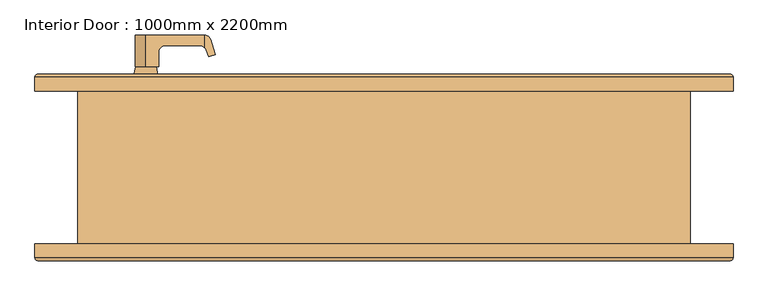
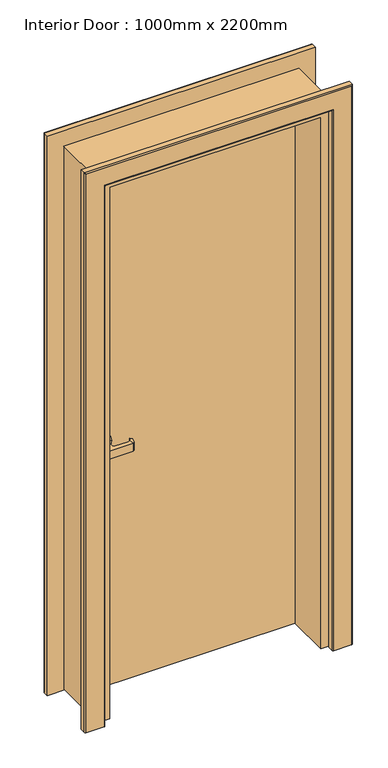
"""IFC4 building model written with IfcOpenShell, lengths in millimetres: door geometry, Interior Door : 1000mm x 2200mm."""

from ifc_helpers import new_model, si_unit, frame, origin, place, context, project, spatial, polyline, circle_curve, ellipse_curve, outline, extrude, faceted_brep, source, transform, mapped, element, save
from ifc_brep_helpers import plane_surface, cylinder_surface, revolved_surface, advanced_brep


def interior_door_1000mm_x_2200mm_5ae40eff(model_context):
    return source(origin(), model_context, "Body", "SolidModel", [
        advanced_brep(
        [(-323.0, 55.325, 910.0), (-377.0, 55.325, 910.0), (-368.0, 55.325, 910.0), (-332.0, 55.325, 910.0), (-349.5, 55.325, 922.0), (-350.5, 55.325, 922.0), (-350.5, 55.325, 898.0), (-349.5, 55.325, 898.0), (-323.0, 58.5, 910.0), (-377.0, 58.5, 910.0), (-332.0, 43.9713587, 910.0), (-368.0, 43.9713587, 910.0), (-349.5, 43.9713587, 898.0), (-350.5, 43.9713587, 898.0), (-350.5, 43.9713587, 922.0), (-349.5, 43.9713587, 922.0)],
        [
            (0, 1, circle_curve(frame((-350.0, 55.325, 910.0), z_axis=(0.0, -1.0, 0.0), x_axis=(-1.0, 0.0, 0.0)), 27.0)),
            (1, 0, circle_curve(frame((-350.0, 55.325, 910.0), z_axis=(0.0, -1.0, 0.0), x_axis=(-1.0, 0.0, 0.0)), 27.0)),
            (2, 3, circle_curve(frame((-350.0, 55.325, 910.0), z_axis=(0.0, 1.0, 0.0), x_axis=(-1.0, 0.0, 0.0)), 18.0)),
            (3, 2, circle_curve(frame((-350.0, 55.325, 910.0), z_axis=(0.0, 1.0, 0.0), x_axis=(-1.0, 0.0, 0.0)), 18.0)),
            (4, 5),
            (5, 6),
            (6, 7),
            (7, 4),
            (8, 9, circle_curve(frame((-350.0, 58.5, 910.0), z_axis=(0.0, 1.0, 0.0), x_axis=(-1.0, 0.0, 0.0)), 27.0)),
            (9, 8, circle_curve(frame((-350.0, 58.5, 910.0), z_axis=(0.0, 1.0, 0.0), x_axis=(-1.0, 0.0, 0.0)), 27.0)),
            (1, 9),
            (8, 0),
            (10, 11, circle_curve(frame((-350.0, 43.9713587, 910.0), z_axis=(0.0, -1.0, 0.0), x_axis=(-1.0, 0.0, 0.0)), 18.0)),
            (11, 10, circle_curve(frame((-350.0, 43.9713587, 910.0), z_axis=(0.0, -1.0, 0.0), x_axis=(-1.0, 0.0, 0.0)), 18.0)),
            (12, 13),
            (13, 14),
            (14, 15),
            (15, 12),
            (11, 2),
            (3, 10),
            (15, 4),
            (7, 12),
            (14, 5),
            (13, 6),
        ],
        [
            plane_surface(frame((-377.0, 55.325, 910.0), z_axis=(0.0, -1.0, 0.0), x_axis=(0.0, 0.0, 1.0))),
            plane_surface(frame((-377.0, 58.5, 910.0), z_axis=(0.0, 1.0, 0.0), x_axis=(0.0, 0.0, -1.0))),
            cylinder_surface(frame((-350.0, 58.5, 910.0), z_axis=(0.0, -1.0, 0.0), x_axis=(-1.0, 0.0, 0.0)), 27.0),
            plane_surface(frame((-368.0, 43.9713587, 910.0), z_axis=(0.0, -1.0, 0.0), x_axis=(0.0, 0.0, 1.0))),
            cylinder_surface(frame((-350.0, 58.5, 910.0), z_axis=(0.0, -1.0, 0.0), x_axis=(-1.0, 0.0, 0.0)), 18.0),
            plane_surface(frame((-349.5, 43.9713587, 898.0), z_axis=(-1.0, 0.0, 0.0), x_axis=(0.0, 1.0, 0.0))),
            plane_surface(frame((-349.5, 43.9713587, 922.0), z_axis=(0.0, 0.0, -1.0), x_axis=(0.0, 1.0, 0.0))),
            plane_surface(frame((-350.5, 43.9713587, 922.0), z_axis=(1.0, 0.0, 0.0), x_axis=(0.0, 1.0, 0.0))),
            plane_surface(frame((-350.5, 43.9713587, 898.0), z_axis=(0.0, 0.0, 1.0), x_axis=(0.0, 1.0, 0.0))),
        ],
        [
            (0, [[1, 2], [3, 4]]),
            (0, [[5, 6, 7, 8]]),
            (1, [[9, 10]]),
            (2, [[11, -9, 12, -2]]),
            (2, [[-12, -10, -11, -1]]),
            (3, [[13, 14], [15, 16, 17, 18]]),
            (4, [[19, -4, 20, -14]]),
            (4, [[-20, -3, -19, -13]]),
            (5, [[21, -8, 22, -18]]),
            (6, [[23, -5, -21, -17]]),
            (7, [[24, -6, -23, -16]]),
            (8, [[-22, -7, -24, -15]]),
        ],
    ),
        advanced_brep(
        [(-323.0, 115.675, 910.0), (-377.0, 115.675, 910.0), (-368.0, 115.675, 910.0), (-332.0, 115.675, 910.0), (-349.5, 115.675, 922.0), (-349.5, 115.675, 898.0), (-350.5, 115.675, 898.0), (-350.5, 115.675, 922.0), (-323.0, 112.5, 910.0), (-377.0, 112.5, 910.0), (-332.0, 127.0286413, 910.0), (-368.0, 127.0286413, 910.0), (-349.5, 127.0286413, 898.0), (-349.5, 127.0286413, 922.0), (-350.5, 127.0286413, 922.0), (-350.5, 127.0286413, 898.0)],
        [
            (0, 1, circle_curve(frame((-350.0, 115.675, 910.0), z_axis=(0.0, 1.0, 0.0), x_axis=(-1.0, 0.0, 0.0)), 27.0)),
            (1, 0, circle_curve(frame((-350.0, 115.675, 910.0), z_axis=(0.0, 1.0, 0.0), x_axis=(-1.0, 0.0, 0.0)), 27.0)),
            (2, 3, circle_curve(frame((-350.0, 115.675, 910.0), z_axis=(0.0, -1.0, 0.0), x_axis=(-1.0, 0.0, 0.0)), 18.0)),
            (3, 2, circle_curve(frame((-350.0, 115.675, 910.0), z_axis=(0.0, -1.0, 0.0), x_axis=(-1.0, 0.0, 0.0)), 18.0)),
            (4, 5),
            (5, 6),
            (6, 7),
            (7, 4),
            (8, 9, circle_curve(frame((-350.0, 112.5, 910.0), z_axis=(0.0, -1.0, 0.0), x_axis=(-1.0, 0.0, 0.0)), 27.0)),
            (9, 8, circle_curve(frame((-350.0, 112.5, 910.0), z_axis=(0.0, -1.0, 0.0), x_axis=(-1.0, 0.0, 0.0)), 27.0)),
            (0, 8),
            (9, 1),
            (10, 11, circle_curve(frame((-350.0, 127.0286413, 910.0), z_axis=(0.0, 1.0, 0.0), x_axis=(-1.0, 0.0, 0.0)), 18.0)),
            (11, 10, circle_curve(frame((-350.0, 127.0286413, 910.0), z_axis=(0.0, 1.0, 0.0), x_axis=(-1.0, 0.0, 0.0)), 18.0)),
            (12, 13),
            (13, 14),
            (14, 15),
            (15, 12),
            (10, 3),
            (2, 11),
            (12, 5),
            (4, 13),
            (7, 14),
            (6, 15),
        ],
        [
            plane_surface(frame((-377.0, 115.675, 910.0), z_axis=(0.0, 1.0, 0.0), x_axis=(0.0, 0.0, 1.0))),
            plane_surface(frame((-377.0, 112.5, 910.0), z_axis=(0.0, -1.0, 0.0), x_axis=(0.0, 0.0, -1.0))),
            cylinder_surface(frame((-350.0, 112.5, 910.0), z_axis=(0.0, 1.0, 0.0), x_axis=(-1.0, 0.0, 0.0)), 27.0),
            plane_surface(frame((-368.0, 127.0286413, 910.0), z_axis=(0.0, 1.0, 0.0), x_axis=(0.0, 0.0, 1.0))),
            cylinder_surface(frame((-350.0, 112.5, 910.0), z_axis=(0.0, 1.0, 0.0), x_axis=(-1.0, 0.0, 0.0)), 18.0),
            plane_surface(frame((-349.5, 127.0286413, 898.0), z_axis=(-1.0, 0.0, 0.0), x_axis=(0.0, -1.0, 0.0))),
            plane_surface(frame((-349.5, 127.0286413, 922.0), z_axis=(0.0, 0.0, -1.0), x_axis=(0.0, -1.0, 0.0))),
            plane_surface(frame((-350.5, 127.0286413, 922.0), z_axis=(1.0, 0.0, 0.0), x_axis=(0.0, -1.0, 0.0))),
            plane_surface(frame((-350.5, 127.0286413, 898.0), z_axis=(0.0, 0.0, 1.0), x_axis=(0.0, -1.0, 0.0))),
        ],
        [
            (0, [[1, 2], [3, 4]]),
            (0, [[5, 6, 7, 8]]),
            (1, [[9, 10]]),
            (2, [[-1, 11, -10, 12]]),
            (2, [[-2, -12, -9, -11]]),
            (3, [[13, 14], [15, 16, 17, 18]]),
            (4, [[-13, 19, -3, 20]]),
            (4, [[-14, -20, -4, -19]]),
            (5, [[-15, 21, -5, 22]]),
            (6, [[-16, -22, -8, 23]]),
            (7, [[-17, -23, -7, 24]]),
            (8, [[-18, -24, -6, -21]]),
        ],
    ),
        advanced_brep(
        [(-305.55, 125.2, 1000.0), (-305.55, 112.5, 1000.0), (-394.45, 112.5, 1000.0), (-394.45, 125.2, 1000.0), (-330.95, 128.375, 1000.0), (-369.05, 128.375, 1000.0), (-350.0, 112.5, 1000.0), (-334.9229513, 148.8140625, 1000.0), (-365.0770487, 148.8140625, 1000.0), (-350.0, 148.8140625, 1000.0)],
        [
            (0, 1),
            (1, 2, circle_curve(frame((-350.0, 112.5, 1000.0), z_axis=(0.0, 1.0, 0.0), x_axis=(-1.0, 0.0, 0.0)), 44.45)),
            (2, 3),
            (3, 0, circle_curve(frame((-350.0, 125.2, 1000.0), z_axis=(0.0, -1.0, 0.0), x_axis=(-1.0, 0.0, 0.0)), 44.45)),
            (2, 1, circle_curve(frame((-350.0, 112.5, 1000.0), z_axis=(0.0, 1.0, 0.0), x_axis=(-1.0, 0.0, 0.0)), 44.45)),
            (0, 3, circle_curve(frame((-350.0, 125.2, 1000.0), z_axis=(0.0, -1.0, 0.0), x_axis=(-1.0, 0.0, 0.0)), 44.45)),
            (4, 0),
            (3, 5),
            (5, 4, circle_curve(frame((-350.0, 128.375, 1000.0), z_axis=(0.0, -1.0, 0.0), x_axis=(-1.0, 0.0, 0.0)), 19.05)),
            (4, 5, circle_curve(frame((-350.0, 128.375, 1000.0), z_axis=(0.0, -1.0, 0.0), x_axis=(-1.0, 0.0, 0.0)), 19.05)),
            (1, 6),
            (6, 2),
            (7, 4),
            (5, 8),
            (8, 7, circle_curve(frame((-350.0, 148.8140625, 1000.0), z_axis=(0.0, -1.0, 0.0), x_axis=(-1.0, 0.0, 0.0)), 15.0770487)),
            (7, 8, circle_curve(frame((-350.0, 148.8140625, 1000.0), z_axis=(0.0, -1.0, 0.0), x_axis=(-1.0, 0.0, 0.0)), 15.0770487)),
            (9, 7),
            (8, 9),
        ],
        [
            cylinder_surface(frame((-350.0, -39.9, 1000.0), z_axis=(0.0, 1.0, 0.0), x_axis=(-1.0, 0.0, 0.0)), 44.45),
            revolved_surface(polyline([(-394.45, 125.2, 1000.0), (-369.05, 128.375, 1000.0)]), (-350.0, -39.9, 1000.0), (0.0, 1.0, 0.0)),
            plane_surface(frame((-350.0, 112.5, 1000.0), z_axis=(0.0, -1.0, 0.0), x_axis=(-1.0, 0.0, 0.0))),
            revolved_surface(polyline([(-369.05, 128.375, 1000.0), (-365.0770487, 148.8140625, 1000.0)]), (-350.0, -39.9, 1000.0), (0.0, 1.0, 0.0)),
            plane_surface(frame((-350.0, 148.8140625, 1000.0), z_axis=(0.0, 1.0, 0.0), x_axis=(-1.0, 0.0, 0.0))),
        ],
        [
            (0, [[1, 2, 3, 4]]),
            (0, [[-3, 5, -1, 6]]),
            (1, [[7, -4, 8, 9]]),
            (1, [[-8, -6, -7, 10]]),
            (2, [[11, 12, -2]]),
            (2, [[-12, -11, -5]]),
            (3, [[13, -9, 14, 15]]),
            (3, [[-14, -10, -13, 16]]),
            (4, [[17, -15, 18]]),
            (4, [[-18, -16, -17]]),
        ],
    ),
        advanced_brep(
        [(-330.95, 169.7736937, 1015.875), (-321.425, 179.2986937, 1015.875), (-270.4853465, 179.2986937, 1015.875), (-264.0071516, 176.7564308, 1015.875), (-264.0071516, 195.05, 1015.875), (-350.0, 195.05, 1015.875), (-350.0, 148.8140625, 1015.875), (-330.95, 148.8140625, 1015.875), (-330.95, 169.7736937, 984.125), (-330.95, 148.8140625, 984.125), (-350.0, 148.8140625, 984.125), (-350.0, 195.05, 984.125), (-264.0071516, 195.05, 984.125), (-264.0071516, 176.7564308, 984.125), (-270.4853465, 179.2986937, 984.125), (-321.425, 179.2986937, 984.125), (-261.5347742, 173.0314356, 984.7111937), (-261.5347742, 173.0314356, 1015.2888063), (-257.8148231, 162.8109537, 985.5931836), (-257.8148231, 162.8109537, 1014.4068164), (-247.6815328, 166.1034593, 987.9957581), (-247.6815328, 166.1034593, 1012.0042419), (-254.9483383, 188.4683869, 986.272819), (-254.9483383, 188.4683869, 1013.727181)],
        [
            (0, 1, circle_curve(frame((-321.425, 169.7736937, 1015.875), z_axis=(0.0, 0.0, -1.0), x_axis=(1.0, 0.0, 0.0)), 9.525)),
            (1, 2),
            (2, 3, circle_curve(frame((-270.4853465, 169.7736937, 1015.875), z_axis=(0.0, 0.0, -1.0), x_axis=(1.0, 0.0, 0.0)), 9.525)),
            (3, 4),
            (4, 5),
            (5, 6),
            (6, 7),
            (7, 0),
            (8, 9),
            (9, 10),
            (10, 11),
            (11, 12),
            (12, 13),
            (13, 14, circle_curve(frame((-270.4853465, 169.7736937, 984.125), z_axis=(0.0, 0.0, 1.0), x_axis=(1.0, 0.0, 0.0)), 9.525)),
            (14, 15),
            (15, 8, circle_curve(frame((-321.425, 169.7736937, 984.125), z_axis=(0.0, 0.0, 1.0), x_axis=(1.0, 0.0, 0.0)), 9.525)),
            (7, 9),
            (8, 0),
            (1, 15),
            (14, 2),
            (11, 5, circle_curve(frame((-350.0, 195.05, 1000.0), z_axis=(0.0, 1.0, 0.0), x_axis=(0.0, 0.0, 1.0)), 15.875)),
            (4, 12),
            (6, 10, circle_curve(frame((-350.0, 148.8140625, 1000.0), z_axis=(0.0, -1.0, 0.0), x_axis=(0.0, 0.0, 1.0)), 15.875)),
            (13, 16, ellipse_curve(frame((-270.4853465, 169.7736937, 982.5890383), z_axis=(0.23070138294863055, 0.0, -0.9730245998460623), x_axis=(0.9730245998460625, 0.0, 0.23070138294862935)), 9.7890639, 9.525)),
            (16, 17),
            (17, 3, ellipse_curve(frame((-270.4853465, 169.7736937, 1017.4109617), z_axis=(0.23070138294863687, 0.0, 0.9730245998460607), x_axis=(-0.9730245998460608, 0.0, 0.23070138294863632)), 9.7890639, 9.525)),
            (16, 18),
            (18, 19),
            (19, 17),
            (18, 20),
            (20, 21),
            (21, 19),
            (20, 22),
            (22, 23),
            (23, 21),
            (4, 23, ellipse_curve(frame((-264.0071516, 185.525, 1015.875), z_axis=(-0.23070138294863687, 0.0, -0.9730245998460607), x_axis=(0.9730245998460608, 0.0, -0.23070138294863632)), 9.7890639, 9.525)),
            (22, 12, ellipse_curve(frame((-264.0071516, 185.525, 984.125), z_axis=(-0.23070138294863055, 0.0, 0.9730245998460623), x_axis=(-0.9730245998460625, 0.0, -0.23070138294862935)), 9.7890639, 9.525)),
        ],
        [
            plane_surface(frame((-311.9, 169.7736937, 1015.875), z_axis=(0.0, 0.0, 1.0), x_axis=(0.0, 1.0, 0.0))),
            plane_surface(frame((-311.9, 169.7736937, 984.125), z_axis=(0.0, 0.0, -1.0), x_axis=(0.0, -1.0, 0.0))),
            plane_surface(frame((-330.95, 148.8140625, 984.125), z_axis=(1.0, 0.0, 0.0), x_axis=(0.0, 0.0, 1.0))),
            plane_surface(frame((-321.425, 179.2986937, 984.125), z_axis=(0.0, -1.0, 0.0), x_axis=(0.0, 0.0, 1.0))),
            plane_surface(frame((-264.0071516, 195.05, 984.125), z_axis=(0.0, 1.0, 0.0), x_axis=(0.0, 0.0, 1.0))),
            plane_surface(frame((-369.05, 148.8140625, 984.125), z_axis=(0.0, -1.0, 0.0), x_axis=(0.0, 0.0, 1.0))),
            revolved_surface(polyline([(-311.90000000000003, 169.7736937, 1015.875), (-311.90000000000003, 169.7736937, 984.125)]), (-321.425, 169.7736937, 1015.875), (0.0, 0.0, 1.0)),
            revolved_surface(polyline([(-260.9603465, 169.7736937, 1019.6693122795026), (-260.9603465, 169.7736937, 980.3306877204975)]), (-270.4853465, 169.7736937, 1015.875), (0.0, 0.0, 1.0)),
            plane_surface(frame((-261.5347742, 173.0314356, 984.125), z_axis=(-0.93969262078591, -0.3420201433256644, 0.0), x_axis=(0.0, 0.0, 1.0))),
            plane_surface(frame((-257.8148231, 162.8109537, 984.125), z_axis=(0.30901699437494523, -0.9510565162951543, 0.0), x_axis=(0.0, 0.0, 1.0))),
            plane_surface(frame((-247.6815328, 166.1034593, 984.125), z_axis=(0.9510565162951542, 0.3090169943749457, 0.0), x_axis=(0.0, 0.0, 1.0))),
            cylinder_surface(frame((-264.0071516, 185.525, 1015.875), z_axis=(0.0, 0.0, -1.0), x_axis=(1.0, 0.0, 0.0)), 9.525),
            cylinder_surface(frame((-350.0, 417.3, 1000.0), z_axis=(0.0, 1.0, 0.0), x_axis=(0.0, 0.0, 1.0)), 15.875),
            plane_surface(frame((-264.0071516, -192.3, 984.125), z_axis=(0.23070138294863055, 0.0, -0.9730245998460623), x_axis=(0.0, 1.0, 0.0))),
            plane_surface(frame((-236.70001, -192.3, 1009.4005539), z_axis=(0.23070138294863687, 0.0, 0.9730245998460607), x_axis=(0.0, 1.0, 0.0))),
        ],
        [
            (0, [[1, 2, 3, 4, 5, 6, 7, 8]]),
            (1, [[9, 10, 11, 12, 13, 14, 15, 16]]),
            (2, [[17, -9, 18, -8]]),
            (3, [[19, -15, 20, -2]]),
            (4, [[-12, 21, -5, 22]]),
            (5, [[-7, 23, -10, -17]]),
            (6, [[-18, -16, -19, -1]]),
            (7, [[-14, 24, 25, 26, -3, -20]]),
            (8, [[27, 28, 29, -25]]),
            (9, [[30, 31, 32, -28]]),
            (10, [[33, 34, 35, -31]]),
            (11, [[36, -34, 37, -22]]),
            (12, [[-21, -11, -23, -6]]),
            (13, [[-37, -33, -30, -27, -24, -13]]),
            (14, [[-26, -29, -32, -35, -36, -4]]),
        ],
    ),
        advanced_brep(
        [(-305.55, 45.8, 1000.0), (-394.45, 45.8, 1000.0), (-394.45, 58.5, 1000.0), (-305.55, 58.5, 1000.0), (-330.95, 42.625, 1000.0), (-369.05, 42.625, 1000.0), (-350.0, 58.5, 1000.0), (-334.9229513, 22.1859375, 1000.0), (-365.0770487, 22.1859375, 1000.0), (-350.0, 22.1859375, 1000.0)],
        [
            (0, 1, circle_curve(frame((-350.0, 45.8, 1000.0), z_axis=(0.0, 1.0, 0.0), x_axis=(-1.0, 0.0, 0.0)), 44.45)),
            (1, 2),
            (2, 3, circle_curve(frame((-350.0, 58.5, 1000.0), z_axis=(0.0, -1.0, 0.0), x_axis=(-1.0, 0.0, 0.0)), 44.45)),
            (3, 0),
            (1, 0, circle_curve(frame((-350.0, 45.8, 1000.0), z_axis=(0.0, 1.0, 0.0), x_axis=(-1.0, 0.0, 0.0)), 44.45)),
            (3, 2, circle_curve(frame((-350.0, 58.5, 1000.0), z_axis=(0.0, -1.0, 0.0), x_axis=(-1.0, 0.0, 0.0)), 44.45)),
            (4, 5, circle_curve(frame((-350.0, 42.625, 1000.0), z_axis=(0.0, 1.0, 0.0), x_axis=(-1.0, 0.0, 0.0)), 19.05)),
            (5, 1),
            (0, 4),
            (5, 4, circle_curve(frame((-350.0, 42.625, 1000.0), z_axis=(0.0, 1.0, 0.0), x_axis=(-1.0, 0.0, 0.0)), 19.05)),
            (2, 6),
            (6, 3),
            (7, 8, circle_curve(frame((-350.0, 22.1859375, 1000.0), z_axis=(0.0, 1.0, 0.0), x_axis=(-1.0, 0.0, 0.0)), 15.0770487)),
            (8, 5),
            (4, 7),
            (8, 7, circle_curve(frame((-350.0, 22.1859375, 1000.0), z_axis=(0.0, 1.0, 0.0), x_axis=(-1.0, 0.0, 0.0)), 15.0770487)),
            (9, 8),
            (7, 9),
        ],
        [
            cylinder_surface(frame((-350.0, 210.9, 1000.0), z_axis=(0.0, -1.0, 0.0), x_axis=(-1.0, 0.0, 0.0)), 44.45),
            revolved_surface(polyline([(-394.45, 45.8, 1000.0), (-369.05, 42.625, 1000.0)]), (-350.0, 210.9, 1000.0), (0.0, -1.0, 0.0)),
            plane_surface(frame((-350.0, 58.5, 1000.0), z_axis=(0.0, 1.0, 0.0), x_axis=(-1.0, 0.0, 0.0))),
            revolved_surface(polyline([(-369.05, 42.625, 1000.0), (-365.0770487, 22.1859375, 1000.0)]), (-350.0, 210.9, 1000.0), (0.0, -1.0, 0.0)),
            plane_surface(frame((-350.0, 22.1859375, 1000.0), z_axis=(0.0, -1.0, 0.0), x_axis=(-1.0, 0.0, 0.0))),
        ],
        [
            (0, [[1, 2, 3, 4]]),
            (0, [[5, -4, 6, -2]]),
            (1, [[7, 8, -1, 9]]),
            (1, [[10, -9, -5, -8]]),
            (2, [[-3, 11, 12]]),
            (2, [[-6, -12, -11]]),
            (3, [[13, 14, -7, 15]]),
            (3, [[16, -15, -10, -14]]),
            (4, [[17, -13, 18]]),
            (4, [[-18, -16, -17]]),
        ],
    ),
        advanced_brep(
        [(-330.95, 1.2263063, 1015.875), (-330.95, 22.1859375, 1015.875), (-350.0, 22.1859375, 1015.875), (-350.0, -24.05, 1015.875), (-264.0071516, -24.05, 1015.875), (-264.0071516, -5.7564308, 1015.875), (-270.4853465, -8.2986937, 1015.875), (-321.425, -8.2986937, 1015.875), (-330.95, 1.2263063, 984.125), (-321.425, -8.2986937, 984.125), (-270.4853465, -8.2986937, 984.125), (-264.0071516, -5.7564308, 984.125), (-264.0071516, -24.05, 984.125), (-350.0, -24.05, 984.125), (-350.0, 22.1859375, 984.125), (-330.95, 22.1859375, 984.125), (-261.5347742, -2.0314356, 1015.2888063), (-261.5347742, -2.0314356, 984.7111937), (-257.8148231, 8.1890463, 1014.4068164), (-257.8148231, 8.1890463, 985.5931836), (-247.6815328, 4.8965407, 1012.0042419), (-247.6815328, 4.8965407, 987.9957581), (-254.9483383, -17.4683869, 1013.727181), (-254.9483383, -17.4683869, 986.272819)],
        [
            (0, 1),
            (1, 2),
            (2, 3),
            (3, 4),
            (4, 5),
            (5, 6, circle_curve(frame((-270.4853465, 1.2263063, 1015.875), z_axis=(0.0, 0.0, -1.0), x_axis=(1.0, 0.0, 0.0)), 9.525)),
            (6, 7),
            (7, 0, circle_curve(frame((-321.425, 1.2263063, 1015.875), z_axis=(0.0, 0.0, -1.0), x_axis=(1.0, 0.0, 0.0)), 9.525)),
            (8, 9, circle_curve(frame((-321.425, 1.2263063, 984.125), z_axis=(0.0, 0.0, 1.0), x_axis=(1.0, 0.0, 0.0)), 9.525)),
            (9, 10),
            (10, 11, circle_curve(frame((-270.4853465, 1.2263063, 984.125), z_axis=(0.0, 0.0, 1.0), x_axis=(1.0, 0.0, 0.0)), 9.525)),
            (11, 12),
            (12, 13),
            (13, 14),
            (14, 15),
            (15, 8),
            (0, 8),
            (15, 1),
            (6, 10),
            (9, 7),
            (12, 4),
            (3, 13, circle_curve(frame((-350.0, -24.05, 1000.0), z_axis=(0.0, -1.0, 0.0), x_axis=(0.0, 0.0, 1.0)), 15.875)),
            (14, 2, circle_curve(frame((-350.0, 22.1859375, 1000.0), z_axis=(0.0, 1.0, 0.0), x_axis=(0.0, 0.0, 1.0)), 15.875)),
            (5, 16, ellipse_curve(frame((-270.4853465, 1.2263063, 1017.4109617), z_axis=(0.23070138294863687, 0.0, 0.9730245998460607), x_axis=(-0.9730245998460608, 0.0, 0.23070138294863632)), 9.7890639, 9.525)),
            (16, 17),
            (17, 11, ellipse_curve(frame((-270.4853465, 1.2263063, 982.5890383), z_axis=(0.23070138294863055, 0.0, -0.9730245998460623), x_axis=(0.9730245998460625, 0.0, 0.23070138294862935)), 9.7890639, 9.525)),
            (16, 18),
            (18, 19),
            (19, 17),
            (18, 20),
            (20, 21),
            (21, 19),
            (20, 22),
            (22, 23),
            (23, 21),
            (12, 23, ellipse_curve(frame((-264.0071516, -14.525, 984.125), z_axis=(-0.23070138294863055, 0.0, 0.9730245998460623), x_axis=(-0.9730245998460625, 0.0, -0.23070138294862935)), 9.7890639, 9.525)),
            (22, 4, ellipse_curve(frame((-264.0071516, -14.525, 1015.875), z_axis=(-0.23070138294863687, 0.0, -0.9730245998460607), x_axis=(0.9730245998460608, 0.0, -0.23070138294863632)), 9.7890639, 9.525)),
        ],
        [
            plane_surface(frame((-311.9, 1.2263063, 1015.875), z_axis=(0.0, 0.0, 1.0), x_axis=(0.0, -1.0, 0.0))),
            plane_surface(frame((-311.9, 1.2263063, 984.125), z_axis=(0.0, 0.0, -1.0), x_axis=(0.0, 1.0, 0.0))),
            plane_surface(frame((-330.95, 22.1859375, 984.125), z_axis=(1.0, 0.0, 0.0), x_axis=(0.0, 0.0, 1.0))),
            plane_surface(frame((-321.425, -8.2986937, 984.125), z_axis=(0.0, 1.0, 0.0), x_axis=(0.0, 0.0, 1.0))),
            plane_surface(frame((-264.0071516, -24.05, 984.125), z_axis=(0.0, -1.0, 0.0), x_axis=(0.0, 0.0, 1.0))),
            plane_surface(frame((-369.05, 22.1859375, 984.125), z_axis=(0.0, 1.0, 0.0), x_axis=(0.0, 0.0, 1.0))),
            revolved_surface(polyline([(-311.90000000000003, 1.2263063, 1015.875), (-311.90000000000003, 1.2263063, 984.125)]), (-321.425, 1.2263063, 1015.875), (0.0, 0.0, 1.0)),
            revolved_surface(polyline([(-260.9603465, 1.2263063, 1019.6693122795026), (-260.9603465, 1.2263063, 980.3306877204975)]), (-270.4853465, 1.2263063, 1015.875), (0.0, 0.0, 1.0)),
            plane_surface(frame((-261.5347742, -2.0314356, 984.125), z_axis=(-0.93969262078591, 0.3420201433256644, 0.0), x_axis=(0.0, 0.0, 1.0))),
            plane_surface(frame((-257.8148231, 8.1890463, 984.125), z_axis=(0.30901699437494523, 0.9510565162951543, 0.0), x_axis=(0.0, 0.0, 1.0))),
            plane_surface(frame((-247.6815328, 4.8965407, 984.125), z_axis=(0.9510565162951542, -0.3090169943749457, 0.0), x_axis=(0.0, 0.0, 1.0))),
            cylinder_surface(frame((-264.0071516, -14.525, 1015.875), z_axis=(0.0, 0.0, -1.0), x_axis=(1.0, 0.0, 0.0)), 9.525),
            cylinder_surface(frame((-350.0, -246.3, 1000.0), z_axis=(0.0, -1.0, 0.0), x_axis=(0.0, 0.0, 1.0)), 15.875),
            plane_surface(frame((-264.0071516, 363.3, 984.125), z_axis=(0.23070138294863055, 0.0, -0.9730245998460623), x_axis=(0.0, -1.0, 0.0))),
            plane_surface(frame((-236.70001, 363.3, 1009.4005539), z_axis=(0.23070138294863687, 0.0, 0.9730245998460607), x_axis=(0.0, -1.0, 0.0))),
        ],
        [
            (0, [[1, 2, 3, 4, 5, 6, 7, 8]]),
            (1, [[9, 10, 11, 12, 13, 14, 15, 16]]),
            (2, [[-1, 17, -16, 18]]),
            (3, [[-7, 19, -10, 20]]),
            (4, [[21, -4, 22, -13]]),
            (5, [[-18, -15, 23, -2]]),
            (6, [[-8, -20, -9, -17]]),
            (7, [[-19, -6, 24, 25, 26, -11]]),
            (8, [[-25, 27, 28, 29]]),
            (9, [[-28, 30, 31, 32]]),
            (10, [[-31, 33, 34, 35]]),
            (11, [[-21, 36, -34, 37]]),
            (12, [[-3, -23, -14, -22]]),
            (13, [[-12, -26, -29, -32, -35, -36]]),
            (14, [[-5, -37, -33, -30, -27, -24]]),
        ],
    ),
        extrude(outline(polyline([(422.0000374, 58.5), (-422.0000374, 58.5), (-422.0000374, 112.5), (422.0000374, 112.5), (422.0000374, 58.5)])), frame((0.0, 0.0, 5.0), z_axis=(0.0, 0.0, 1.0), x_axis=(1.0, 0.0, 0.0)), (0.0, 0.0, 1.0), 2167.0000374),
        faceted_brep([(-405.0000128, 58.5, 5.0), (-405.0000128, -112.5, 5.0), (-450.0, -112.5, 5.0), (-450.0, 112.5, 5.0), (-422.0000374, 112.5, 5.0), (-422.0000374, 58.5, 5.0), (-405.0000128, 58.5, 2155.0000128), (-405.0000128, -112.5, 2155.0000128), (405.0000128, -112.5, 2155.0000128), (405.0000128, -112.5, 5.0), (450.0, -112.5, 5.0), (450.0, -112.5, 2200.0), (-450.0, -112.5, 2200.0), (-450.0, 112.5, 2200.0), (450.0, 112.5, 2200.0), (450.0, 112.5, 5.0), (422.0000374, 112.5, 5.0), (422.0000374, 112.5, 2172.0000374), (-422.0000374, 112.5, 2172.0000374), (-422.0000374, 58.5, 2172.0000374), (422.0000374, 58.5, 2172.0000374), (422.0000374, 58.5, 5.0), (405.0000128, 58.5, 5.0), (405.0000128, 58.5, 2155.0000128)], [[[0, 1, 2, 3, 4, 5]], [[0, 6, 7, 1]], [[2, 1, 7, 8, 9, 10, 11, 12]], [[3, 2, 12, 13]], [[4, 3, 13, 14, 15, 16, 17, 18]], [[5, 4, 18, 19]], [[0, 5, 19, 20, 21, 22, 23, 6]], [[8, 23, 22, 9]], [[9, 22, 21, 16, 15, 10]], [[14, 11, 10, 15]], [[20, 17, 16, 21]], [[13, 12, 11, 14]], [[19, 18, 17, 20]], [[7, 6, 23, 8]]]),
        advanced_brep(
        [(-439.9983436, 137.5, 0.0), (-435.0, 132.5016564, 0.0), (-435.0, 112.5, 0.0), (-512.9993919, 112.5, 0.0), (-512.9993919, 132.4992678, 0.0), (-507.9986597, 137.5, 0.0), (-439.9983436, 137.5, 2189.9983436), (-435.0, 132.5016564, 2185.0), (-435.0, 112.5, 2185.0), (435.0, 112.5, 2185.0), (435.0, 112.5, 0.0), (512.9993919, 112.5, 0.0), (512.9993919, 112.5, 2262.9993919), (-512.9993919, 112.5, 2262.9993919), (-512.9993919, 132.4992678, 2262.9993919), (-507.9986597, 137.5, 2257.9986597), (507.9986597, 137.5, 2257.9986597), (507.9986597, 137.5, 0.0), (439.9983436, 137.5, 0.0), (439.9983436, 137.5, 2189.9983436), (435.0, 132.5016564, 2185.0), (435.0, 132.5016564, 0.0), (512.9993919, 132.4992678, 0.0), (512.9993919, 132.4992678, 2262.9993919)],
        [
            (0, 1, circle_curve(frame((-439.9983436, 132.5016564, 0.0), z_axis=(0.0, 0.0, -1.0), x_axis=(-1.0, 0.0, 0.0)), 4.9983436)),
            (1, 2),
            (2, 3),
            (3, 4),
            (4, 5, circle_curve(frame((-507.9986597, 132.4992678, 0.0), z_axis=(0.0, 0.0, -1.0), x_axis=(-1.0, 0.0, 0.0)), 5.0007322)),
            (5, 0),
            (0, 6),
            (6, 7, ellipse_curve(frame((-439.9983436, 132.5016564, 2189.9983436), z_axis=(-0.7071067811865475, 0.0, -0.7071067811865475), x_axis=(0.7071067811865474, 0.0, -0.7071067811865476)), 7.0687253, 4.9983436)),
            (7, 1),
            (7, 8),
            (8, 2),
            (8, 9),
            (9, 10),
            (10, 11),
            (11, 12),
            (12, 13),
            (13, 3),
            (13, 14),
            (14, 4),
            (14, 15, ellipse_curve(frame((-507.9986597, 132.4992678, 2257.9986597), z_axis=(-0.7071067811865475, 0.0, -0.7071067811865475), x_axis=(0.7071067811865474, 0.0, -0.7071067811865476)), 7.0721032, 5.0007322)),
            (15, 5),
            (15, 16),
            (16, 17),
            (17, 18),
            (18, 19),
            (19, 6),
            (9, 20),
            (20, 21),
            (21, 10),
            (17, 22, circle_curve(frame((507.9986597, 132.4992678, 0.0), z_axis=(0.0, 0.0, -1.0), x_axis=(1.0, 0.0, 0.0)), 5.0007322)),
            (22, 11),
            (21, 18, circle_curve(frame((439.9983436, 132.5016564, 0.0), z_axis=(0.0, 0.0, -1.0), x_axis=(1.0, 0.0, 0.0)), 4.9983436)),
            (23, 12),
            (22, 23),
            (16, 23, ellipse_curve(frame((507.9986597, 132.4992678, 2257.9986597), z_axis=(0.7071067811865475, 0.0, -0.7071067811865475), x_axis=(0.7071067811865474, 0.0, 0.7071067811865476)), 7.0721032, 5.0007322)),
            (20, 19, ellipse_curve(frame((439.9983436, 132.5016564, 2189.9983436), z_axis=(0.7071067811865475, 0.0, -0.7071067811865475), x_axis=(0.7071067811865474, 0.0, 0.7071067811865476)), 7.0687253, 4.9983436)),
            (20, 7),
            (23, 14),
        ],
        [
            plane_surface(frame((-450.0, -125.0, 0.0), z_axis=(0.0, 0.0, -1.0), x_axis=(0.0, -1.0, 0.0))),
            cylinder_surface(frame((-439.9983436, 132.5016564, 0.0), z_axis=(0.0, 0.0, -1.0), x_axis=(-1.0, 0.0, 0.0)), 4.9983436),
            plane_surface(frame((-435.0, 132.5016564, 0.0), z_axis=(1.0, 0.0, 0.0), x_axis=(0.0, 0.0, 1.0))),
            plane_surface(frame((-435.0, 112.5, 0.0), z_axis=(0.0, -1.0, 0.0), x_axis=(0.0, 0.0, 1.0))),
            plane_surface(frame((-512.9993919, 112.5, 0.0), z_axis=(-1.0, 0.0, 0.0), x_axis=(0.0, 0.0, 1.0))),
            cylinder_surface(frame((-507.9986597, 132.4992678, 0.0), z_axis=(0.0, 0.0, -1.0), x_axis=(-1.0, 0.0, 0.0)), 5.0007322),
            plane_surface(frame((-507.9986597, 137.5, 0.0), z_axis=(0.0, 1.0, 0.0), x_axis=(0.0, 0.0, 1.0))),
            plane_surface(frame((435.0, 132.5016564, 2185.0), z_axis=(-1.0, 0.0, 0.0), x_axis=(0.0, 0.0, -1.0))),
            plane_surface(frame((450.0, -125.0, 0.0), z_axis=(0.0, 0.0, -1.0), x_axis=(0.0, -1.0, 0.0))),
            plane_surface(frame((512.9993919, 112.5, 2262.9993919), z_axis=(1.0, 0.0, 0.0), x_axis=(0.0, 0.0, -1.0))),
            cylinder_surface(frame((507.9986597, 132.4992678, 2200.0), z_axis=(0.0, 0.0, 1.0), x_axis=(1.0, 0.0, 0.0)), 5.0007322),
            cylinder_surface(frame((439.9983436, 132.5016564, 2200.0), z_axis=(0.0, 0.0, 1.0), x_axis=(1.0, 0.0, 0.0)), 4.9983436),
            cylinder_surface(frame((-450.0, 132.5016564, 2189.9983436), z_axis=(-1.0, 0.0, 0.0), x_axis=(0.0, 0.0, 1.0)), 4.9983436),
            plane_surface(frame((-435.0, 132.5016564, 2185.0), z_axis=(0.0, 0.0, -1.0), x_axis=(1.0, 0.0, 0.0))),
            plane_surface(frame((-512.9993919, 112.5, 2262.9993919), z_axis=(0.0, 0.0, 1.0), x_axis=(1.0, 0.0, 0.0))),
            cylinder_surface(frame((-450.0, 132.4992678, 2257.9986597), z_axis=(-1.0, 0.0, 0.0), x_axis=(0.0, 0.0, 1.0)), 5.0007322),
        ],
        [
            (0, [[1, 2, 3, 4, 5, 6]]),
            (1, [[-1, 7, 8, 9]]),
            (2, [[-2, -9, 10, 11]]),
            (3, [[-3, -11, 12, 13, 14, 15, 16, 17]]),
            (4, [[-4, -17, 18, 19]]),
            (5, [[-5, -19, 20, 21]]),
            (6, [[-6, -21, 22, 23, 24, 25, 26, -7]]),
            (7, [[27, 28, 29, -13]]),
            (8, [[-24, 30, 31, -14, -29, 32]]),
            (9, [[33, -15, -31, 34]]),
            (10, [[35, -34, -30, -23]]),
            (11, [[36, -25, -32, -28]]),
            (12, [[-8, -26, -36, 37]]),
            (13, [[-10, -37, -27, -12]]),
            (14, [[-18, -16, -33, 38]]),
            (15, [[-20, -38, -35, -22]]),
        ],
    ),
        advanced_brep(
        [(-439.9983436, -137.5, 0.0), (-507.9986597, -137.5, 0.0), (-512.9993919, -132.4992678, 0.0), (-512.9993919, -112.5, 0.0), (-435.0, -112.5, 0.0), (-435.0, -132.5016564, 0.0), (-439.9983436, -137.5, 2189.9983436), (439.9983436, -137.5, 2189.9983436), (439.9983436, -137.5, 0.0), (507.9986597, -137.5, 0.0), (507.9986597, -137.5, 2257.9986597), (-507.9986597, -137.5, 2257.9986597), (-512.9993919, -132.4992678, 2262.9993919), (-512.9993919, -112.5, 2262.9993919), (512.9993919, -112.5, 2262.9993919), (512.9993919, -112.5, 0.0), (435.0, -112.5, 0.0), (435.0, -112.5, 2185.0), (-435.0, -112.5, 2185.0), (-435.0, -132.5016564, 2185.0), (512.9993919, -132.4992678, 2262.9993919), (512.9993919, -132.4992678, 0.0), (435.0, -132.5016564, 0.0), (435.0, -132.5016564, 2185.0)],
        [
            (0, 1),
            (1, 2, circle_curve(frame((-507.9986597, -132.4992678, 0.0), z_axis=(0.0, 0.0, -1.0), x_axis=(1.0, 0.0, 0.0)), 5.0007322)),
            (2, 3),
            (3, 4),
            (4, 5),
            (5, 0, circle_curve(frame((-439.9983436, -132.5016564, 0.0), z_axis=(0.0, 0.0, -1.0), x_axis=(1.0, 0.0, 0.0)), 4.9983436)),
            (0, 6),
            (6, 7),
            (7, 8),
            (8, 9),
            (9, 10),
            (10, 11),
            (11, 1),
            (11, 12, ellipse_curve(frame((-507.9986597, -132.4992678, 2257.9986597), z_axis=(-0.7071067811865475, 0.0, -0.7071067811865475), x_axis=(0.7071067811865474, 0.0, -0.7071067811865476)), 7.0721032, 5.0007322)),
            (12, 2),
            (12, 13),
            (13, 3),
            (13, 14),
            (14, 15),
            (15, 16),
            (16, 17),
            (17, 18),
            (18, 4),
            (18, 19),
            (19, 5),
            (19, 6, ellipse_curve(frame((-439.9983436, -132.5016564, 2189.9983436), z_axis=(-0.7071067811865475, 0.0, -0.7071067811865475), x_axis=(0.7071067811865474, 0.0, -0.7071067811865476)), 7.0687253, 4.9983436)),
            (14, 20),
            (20, 21),
            (21, 15),
            (8, 22, circle_curve(frame((439.9983436, -132.5016564, 0.0), z_axis=(0.0, 0.0, -1.0), x_axis=(-1.0, 0.0, 0.0)), 4.9983436)),
            (22, 16),
            (21, 9, circle_curve(frame((507.9986597, -132.4992678, 0.0), z_axis=(0.0, 0.0, -1.0), x_axis=(-1.0, 0.0, 0.0)), 5.0007322)),
            (23, 17),
            (22, 23),
            (7, 23, ellipse_curve(frame((439.9983436, -132.5016564, 2189.9983436), z_axis=(0.7071067811865475, 0.0, -0.7071067811865475), x_axis=(0.7071067811865474, 0.0, 0.7071067811865476)), 7.0687253, 4.9983436)),
            (20, 10, ellipse_curve(frame((507.9986597, -132.4992678, 2257.9986597), z_axis=(0.7071067811865475, 0.0, -0.7071067811865475), x_axis=(0.7071067811865474, 0.0, 0.7071067811865476)), 7.0721032, 5.0007322)),
            (19, 23),
            (12, 20),
        ],
        [
            plane_surface(frame((-450.0, 125.0, 0.0), z_axis=(0.0, 0.0, -1.0), x_axis=(0.0, 1.0, 0.0))),
            plane_surface(frame((-439.9983436, -137.5, 0.0), z_axis=(0.0, -1.0, 0.0), x_axis=(0.0, 0.0, 1.0))),
            cylinder_surface(frame((-507.9986597, -132.4992678, 0.0), z_axis=(0.0, 0.0, -1.0), x_axis=(1.0, 0.0, 0.0)), 5.0007322),
            plane_surface(frame((-512.9993919, -132.4992678, 0.0), z_axis=(-1.0, 0.0, 0.0), x_axis=(0.0, 0.0, 1.0))),
            plane_surface(frame((-512.9993919, -112.5, 0.0), z_axis=(0.0, 1.0, 0.0), x_axis=(0.0, 0.0, 1.0))),
            plane_surface(frame((-435.0, -112.5, 0.0), z_axis=(1.0, 0.0, 0.0), x_axis=(0.0, 0.0, 1.0))),
            cylinder_surface(frame((-439.9983436, -132.5016564, 0.0), z_axis=(0.0, 0.0, -1.0), x_axis=(1.0, 0.0, 0.0)), 4.9983436),
            plane_surface(frame((512.9993919, -132.4992678, 2262.9993919), z_axis=(1.0, 0.0, 0.0), x_axis=(0.0, 0.0, -1.0))),
            plane_surface(frame((450.0, 125.0, 0.0), z_axis=(0.0, 0.0, -1.0), x_axis=(0.0, 1.0, 0.0))),
            plane_surface(frame((435.0, -112.5, 2185.0), z_axis=(-1.0, 0.0, 0.0), x_axis=(0.0, 0.0, -1.0))),
            cylinder_surface(frame((439.9983436, -132.5016564, 2200.0), z_axis=(0.0, 0.0, 1.0), x_axis=(-1.0, 0.0, 0.0)), 4.9983436),
            cylinder_surface(frame((507.9986597, -132.4992678, 2200.0), z_axis=(0.0, 0.0, 1.0), x_axis=(-1.0, 0.0, 0.0)), 5.0007322),
            cylinder_surface(frame((-450.0, -132.5016564, 2189.9983436), z_axis=(-1.0, 0.0, 0.0), x_axis=(0.0, 0.0, -1.0)), 4.9983436),
            plane_surface(frame((-435.0, -112.5, 2185.0), z_axis=(0.0, 0.0, -1.0), x_axis=(1.0, 0.0, 0.0))),
            plane_surface(frame((-512.9993919, -132.4992678, 2262.9993919), z_axis=(0.0, 0.0, 1.0), x_axis=(1.0, 0.0, 0.0))),
            cylinder_surface(frame((-450.0, -132.4992678, 2257.9986597), z_axis=(-1.0, 0.0, 0.0), x_axis=(0.0, 0.0, -1.0)), 5.0007322),
        ],
        [
            (0, [[1, 2, 3, 4, 5, 6]]),
            (1, [[-1, 7, 8, 9, 10, 11, 12, 13]]),
            (2, [[-2, -13, 14, 15]]),
            (3, [[-3, -15, 16, 17]]),
            (4, [[-4, -17, 18, 19, 20, 21, 22, 23]]),
            (5, [[-5, -23, 24, 25]]),
            (6, [[-6, -25, 26, -7]]),
            (7, [[27, 28, 29, -19]]),
            (8, [[30, 31, -20, -29, 32, -10]]),
            (9, [[33, -21, -31, 34]]),
            (10, [[35, -34, -30, -9]]),
            (11, [[36, -11, -32, -28]]),
            (12, [[-26, 37, -35, -8]]),
            (13, [[-24, -22, -33, -37]]),
            (14, [[-16, 38, -27, -18]]),
            (15, [[-14, -12, -36, -38]]),
        ],
    ),
    ])


if __name__ == "__main__":
    model = new_model("IFC4")
    model_context = context("Model", 3, world=origin())
    ifc_project = project(units=[si_unit("LENGTHUNIT", "METRE", prefix="MILLI")], contexts=[model_context])
    site = spatial("IfcSite", under=ifc_project)
    building = spatial("IfcBuilding", under=site)
    placement = place(None, origin())
    interior_door_1000mm_x_2200mm_shape = interior_door_1000mm_x_2200mm_5ae40eff(model_context)
    element("IfcDoor", 1, ObjectType="Interior Door : 1000mm x 2200mm", at=placement, inside=building, context=model_context, shape_type="MappedRepresentation", body=[
        mapped(interior_door_1000mm_x_2200mm_shape, transform((0.0, 0.0, 0.0), x_axis=(1.0, 0.0, 0.0), y_axis=(0.0, 1.0, 0.0), z_axis=(0.0, 0.0, 1.0))),
    ])
    save(model, "model.ifc")

# Revit data of these elements
# Type "Interior Door : 1000mm x 2200mm"
#   Type Mark = "46"
#   Panel Type = ""
#   Location [instance default] = ""
#   Door Type = "Semi Solid Flushed Wooden Door Bed Room Entrance"
#   Construction Type Id = "DOOR"
#   Analytic Construction = "Wooden"
#   Thickness = 54 mm
#   Thermal Resistance (R) = 0.4557 (m²·K)/W
#   Heat Transfer Coefficient (U) = 2.1944 W/(m²·K)
#   Height = 2200 mm
#   Trim Projection Ext = 25 mm
#   Trim Projection Int = 25 mm
#   Width = 900 mm
#   Define Thermal Properties by = 1
#   Threshold Material = BEL-Threshold material-Marble
#   Jamb Material = BEL-Jamb material- Dark stained african solid teakwood
#   Door Material = BEL-Panel material- Dark stained african teakwood veneer
#   Frame Material = BEL-Frame material- Dark stained african teakwood
#   Visual Light Transmittance = 0
#   Solar Heat Gain Coefficient = 0
#   Function = (empty or 0)
#   Wall Closure = (empty or 0)
# Element 1 (IfcDoor, "Interior Door : 1000mm x 2200mm")
#   Materials on its faces: "Metal - IR - Satin Chrome", "BEL-Frame material- Dark stained african teakwood", "BEL-Jamb material- Dark stained african solid teakwood", "BEL-Panel material- Dark stained african teakwood veneer"
# Materials
#   "BEL-Threshold material-Marble": class "Unassigned", colour RGB 197 197 199, transparency 0, Cost = 0
#   "BEL-Jamb material- Dark stained african solid teakwood": class "Wood", colour RGB 131 77 56, transparency 0, Description = "Dark stained African teakwood", Cost = 0
#   "BEL-Panel material- Dark stained african teakwood veneer": class "Wood", colour RGB 131 77 56, transparency 0, Description = "Dark stained African teakwood", Cost = 0
#   "BEL-Frame material- Dark stained african teakwood": class "Wood", colour RGB 89 52 38, transparency 0, Description = "Dark stained African teakwood", Cost = 0
#   "Metal - IR - Satin Chrome": class "Miscellaneous", colour RGB 244 244 244, transparency 0, Cost = 0
